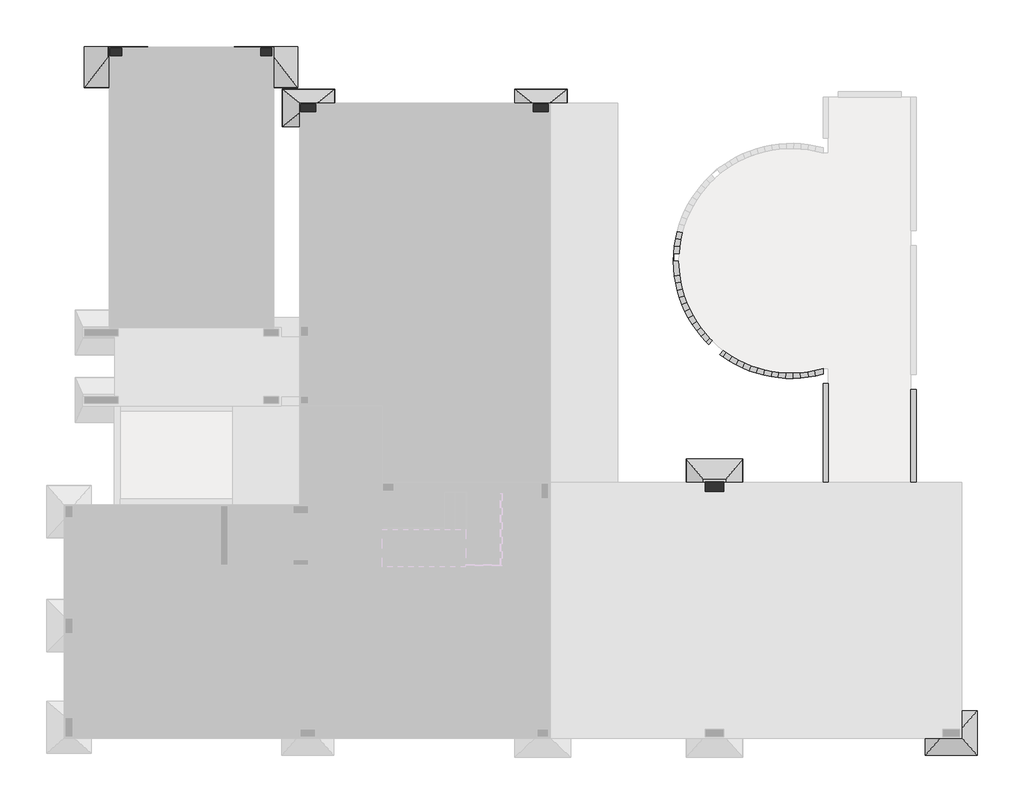
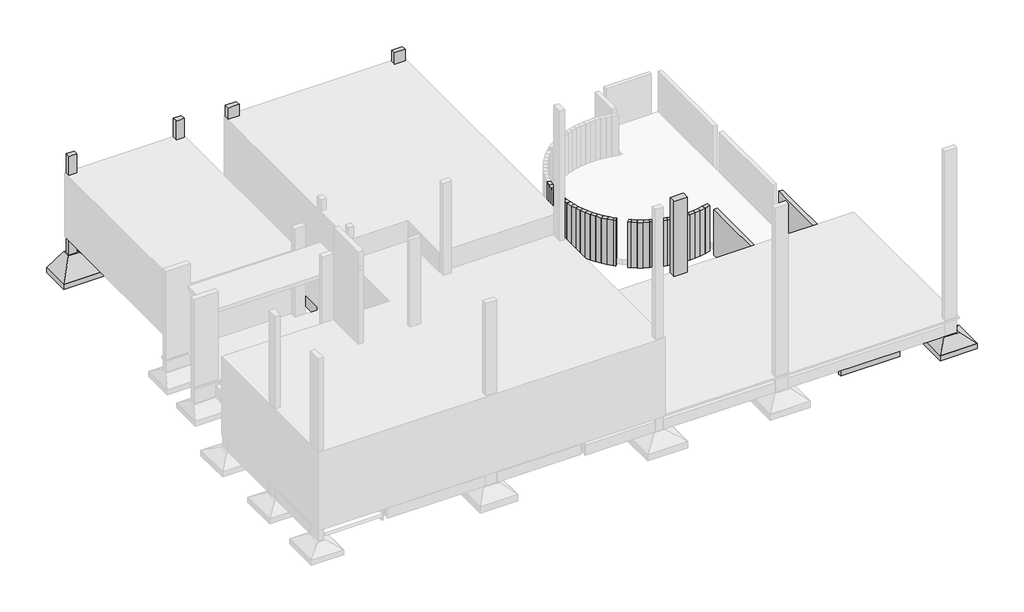
# One storey, part 3 of 4: 37 beams, 7 fasteners, 5 columns.
"""IFC4 building model written with IfcOpenShell, lengths in millimetres."""

import ifcopenshell
import ifcopenshell.guid

model = None  # the IFC model being written
_history = None  # IfcOwnerHistory: only IFC2X3 demands one
_inside = {}  # id of a spatial element -> (the spatial element, [elements in it])
_under = {}  # id of a project, library or spatial element -> (it, [spatial elements below it])
_declared = {}  # id of a project -> (the project, [libraries it declares])
_typed = {}  # id of a type object -> (the type object, [elements of that type])
_made_of = {}  # id of a material, layer set ... -> (it, [elements and type objects made of it])


def new_model(schema):
    """Start an empty IFC model of exactly this schema.

    Asked for "IFC4X3", IfcOpenShell would pick the latest addendum, in which some entities
    have other attributes; the version numbers below select the first issue.
    IFC2X3 requires an IfcOwnerHistory on every rooted entity: one is made here for all.
    """
    global model, _history
    if schema == "IFC4X3":
        model = ifcopenshell.file(schema_version=(4, 3, 0, 0))
    else:
        model = ifcopenshell.file(schema=schema)
    _inside.clear()
    _under.clear()
    _declared.clear()
    _typed.clear()
    _made_of.clear()
    _history = None
    if model.schema == "IFC2X3":
        org = make("IfcOrganization", Name="unknown")
        user = make(
            "IfcPersonAndOrganization",
            ThePerson=make("IfcPerson", FamilyName="unknown"),
            TheOrganization=org,
        )
        app = make(
            "IfcApplication",
            ApplicationDeveloper=org,
            Version="unknown",
            ApplicationFullName="unknown",
            ApplicationIdentifier="unknown",
        )
        _history = make(
            "IfcOwnerHistory",
            OwningUser=user,
            OwningApplication=app,
            ChangeAction="ADDED",
            CreationDate=0,
        )
    return model


def make(cls, **values):
    """One entity of the class cls with the attributes given. An attribute that is None is left unset."""
    return model.create_entity(
        cls, **{name: value for name, value in values.items() if value is not None}
    )


def rooted(cls, **values):
    """An entity with a GlobalId (a new one), such as an element, a storey or a relation."""
    return make(cls, GlobalId=ifcopenshell.guid.new(), OwnerHistory=_history, **values)


def si_unit(unit_type, name, prefix=None):
    """IfcSIUnit, for example si_unit("LENGTHUNIT", "METRE", prefix="MILLI")."""
    return make("IfcSIUnit", UnitType=unit_type, Prefix=prefix, Name=name)


def assignment(units):
    """IfcUnitAssignment: the units of a project."""
    return None if units is None else make("IfcUnitAssignment", Units=units)


def point(xyz):
    """IfcCartesianPoint."""
    return None if xyz is None else make("IfcCartesianPoint", Coordinates=xyz)


def direction(xyz):
    """IfcDirection."""
    return None if xyz is None else make("IfcDirection", DirectionRatios=xyz)


def frame(location, z_axis=None, x_axis=None):
    """IfcAxis2Placement3D, a coordinate frame: its origin and axes. An axis left out is left unset."""
    return make(
        "IfcAxis2Placement3D",
        Location=point(location),
        Axis=direction(z_axis),
        RefDirection=direction(x_axis),
    )


def frame_2d(location, x_axis=None):
    """IfcAxis2Placement2D, a coordinate frame in the plane: its origin and x axis."""
    return make(
        "IfcAxis2Placement2D", Location=point(location), RefDirection=direction(x_axis)
    )


def origin():
    """The frame at (0, 0, 0) with its axes left unset."""
    return frame((0.0, 0.0, 0.0))


def place(relative_to, where):
    """IfcLocalPlacement: puts the frame where relative to a parent placement (None: the world)."""
    return make(
        "IfcLocalPlacement", PlacementRelTo=relative_to, RelativePlacement=where
    )


def context(
    kind, dimensions, precision=None, world=None, true_north=None, identifier=None
):
    """IfcGeometricRepresentationContext, for example the 3D "Model" context."""
    return make(
        "IfcGeometricRepresentationContext",
        ContextIdentifier=identifier,
        ContextType=kind,
        CoordinateSpaceDimension=dimensions,
        Precision=precision,
        WorldCoordinateSystem=world,
        TrueNorth=true_north,
    )


def project(units=None, contexts=None):
    """IfcProject with its units and contexts."""
    return rooted(
        "IfcProject",
        Name="project",
        RepresentationContexts=contexts,
        UnitsInContext=assignment(units),
    )


def spatial(cls, under=None, at=None, **own):
    """A site, building, storey or space (cls), placed at a placement, below another one or the project."""
    s = rooted(cls, ObjectPlacement=at, **own)
    if under is not None:
        _under.setdefault(under.id(), (under, []))[1].append(s)
    return s


def polyline(points):
    """IfcPolyline through the points."""
    return make("IfcPolyline", Points=[point(p) for p in points])


def circle_curve(where, radius):
    """IfcCircle in the frame where."""
    return make("IfcCircle", Position=where, Radius=radius)


def trimmed(basis, trim1, trim2, sense, master):
    """IfcTrimmedCurve: the piece of a basis curve between two trims."""
    return make(
        "IfcTrimmedCurve",
        BasisCurve=basis,
        Trim1=trim1,
        Trim2=trim2,
        SenseAgreement=sense,
        MasterRepresentation=master,
    )


def segment(curve, same_sense, transition):
    """IfcCompositeCurveSegment."""
    return make(
        "IfcCompositeCurveSegment",
        Transition=transition,
        SameSense=same_sense,
        ParentCurve=curve,
    )


def composite_curve(segments, self_intersect=None):
    """IfcCompositeCurve: segments joined end to end."""
    return make("IfcCompositeCurve", Segments=segments, SelfIntersect=self_intersect)


def outline(outer, holes=None, kind="AREA"):
    """IfcArbitraryClosedProfileDef: a profile drawn as a closed curve; with holes, ...WithVoids."""
    if holes is None:
        return make("IfcArbitraryClosedProfileDef", ProfileType=kind, OuterCurve=outer)
    return make(
        "IfcArbitraryProfileDefWithVoids",
        ProfileType=kind,
        OuterCurve=outer,
        InnerCurves=holes,
    )


def extrude(swept, where, along, depth):
    """IfcExtrudedAreaSolid: the profile swept, set in the frame where, extruded along a direction by depth."""
    return make(
        "IfcExtrudedAreaSolid",
        SweptArea=swept,
        Position=where,
        ExtrudedDirection=direction(along),
        Depth=depth,
    )


def faces_of(points, faces, orient=None, outer=None):
    """IfcFace entities. A face is a list of loops; a loop is a list of indices into points, from 0.

    orient and outer hold one flag for each loop. By default every Orientation is true, the
    first loop of a face is its IfcFaceOuterBound and the others are IfcFaceBound.
    """
    made = []
    for i, loops in enumerate(faces):
        bounds = []
        for j, loop in enumerate(loops):
            is_outer = j == 0 if outer is None else outer[i][j]
            bounds.append(
                make(
                    "IfcFaceOuterBound" if is_outer else "IfcFaceBound",
                    Bound=make("IfcPolyLoop", Polygon=[points[k] for k in loop]),
                    Orientation=True if orient is None else orient[i][j],
                )
            )
        made.append(make("IfcFace", Bounds=bounds))
    return made


def faceted_brep(points, faces, orient=None, outer=None, voids=None):
    """IfcFacetedBrep: a solid bounded by flat faces; with voids (closed shells), ...WithVoids."""
    shared = [point(p) for p in points]
    hull = make("IfcClosedShell", CfsFaces=faces_of(shared, faces, orient, outer))
    if voids is None:
        return make("IfcFacetedBrep", Outer=hull)
    return make(
        "IfcFacetedBrepWithVoids",
        Outer=hull,
        Voids=[
            make(cls, CfsFaces=faces_of(shared, fs, o, b)) for cls, fs, o, b in voids
        ],
    )


def shape(context_of_items, identifier, shape_type, items):
    """IfcShapeRepresentation: the items that make up one representation, for example the "Body"."""
    return make(
        "IfcShapeRepresentation",
        ContextOfItems=context_of_items,
        RepresentationIdentifier=identifier,
        RepresentationType=shape_type,
        Items=items,
    )


def source(mapping_origin, context_of_items, identifier, shape_type, items):
    """IfcRepresentationMap: a shape defined once, which mapped items show again and again."""
    return make(
        "IfcRepresentationMap",
        MappingOrigin=mapping_origin,
        MappedRepresentation=shape(context_of_items, identifier, shape_type, items),
    )


def transform(
    local_origin,
    x_axis=None,
    y_axis=None,
    z_axis=None,
    scale=None,
    scale2=None,
    scale3=None,
    uniform=True,
):
    """IfcCartesianTransformationOperator3D, or its non-uniform kind. x_axis, y_axis, z_axis: its Axis1, 2, 3."""
    if uniform:
        return make(
            "IfcCartesianTransformationOperator3D",
            Axis1=direction(x_axis),
            Axis2=direction(y_axis),
            LocalOrigin=point(local_origin),
            Scale=scale,
            Axis3=direction(z_axis),
        )
    return make(
        "IfcCartesianTransformationOperator3DnonUniform",
        Axis1=direction(x_axis),
        Axis2=direction(y_axis),
        LocalOrigin=point(local_origin),
        Scale=scale,
        Axis3=direction(z_axis),
        Scale2=scale2,
        Scale3=scale3,
    )


def mapped(mapping_source, mapping_target):
    """IfcMappedItem: shows the shape of a source again, moved by a transform."""
    return make(
        "IfcMappedItem", MappingSource=mapping_source, MappingTarget=mapping_target
    )


def made_of(thing, what):
    """Note that an element or type object is made of a material, layer set ...; save() writes the relation."""
    if what is not None:
        _made_of.setdefault(what.id(), (what, []))[1].append(thing)
    return thing


def element(
    cls,
    number,
    at=None,
    inside=None,
    cuts=None,
    type_object=None,
    material=None,
    context=None,
    identifier="Body",
    shape_type=None,
    held_by="IfcProductDefinitionShape",
    body=None,
    shapes=None,
    **own,
):
    """One element of the class cls, such as IfcWall. Its Tag is "e" and its number.

    at: its placement. inside: the storey or other place that contains it. cuts: it is an
    opening in that element (IfcRelVoidsElement). A single representation is given by context,
    identifier, shape_type and body (its items); several are given by shapes. held_by: the class
    of the entity that holds the representations. save() writes the other relations.
    """
    e = rooted(cls, Tag="e%d" % number, ObjectPlacement=at, **own)
    if body is not None:
        shapes = [shape(context, identifier, shape_type, body)]
    if shapes is not None:
        e.Representation = make(held_by, Representations=shapes)
    if inside is not None:
        _inside.setdefault(inside.id(), (inside, []))[1].append(e)
    if cuts is not None:
        rooted(
            "IfcRelVoidsElement", RelatingBuildingElement=cuts, RelatedOpeningElement=e
        )
    if type_object is not None:
        _typed.setdefault(type_object.id(), (type_object, []))[1].append(e)
    return made_of(e, material)


def aggregate(whole, parts):
    """IfcRelAggregates: a whole, such as a stair, and the parts it consists of."""
    return rooted("IfcRelAggregates", RelatingObject=whole, RelatedObjects=parts)


def save(model, path):
    """Write the relations noted so far, then the file.

    IfcRelAggregates (storeys below a building ...), IfcRelContainedInSpatialStructure (elements
    in a storey), IfcRelDefinesByType, IfcRelAssociatesMaterial and IfcRelDeclares: one each for
    every whole, place, type object, material and project.
    """
    for whole, parts in _under.values():
        aggregate(whole, parts)
    for where, things in _inside.values():
        rooted(
            "IfcRelContainedInSpatialStructure",
            RelatedElements=things,
            RelatingStructure=where,
        )
    for kind, things in _typed.values():
        rooted("IfcRelDefinesByType", RelatedObjects=things, RelatingType=kind)
    for what, things in _made_of.values():
        rooted("IfcRelAssociatesMaterial", RelatedObjects=things, RelatingMaterial=what)
    for by, libraries in _declared.values():
        rooted("IfcRelDeclares", RelatingContext=by, RelatedDefinitions=libraries)
    model.write(path)


def tqs_viga_retangular_19_0_x_30_0_29604a85(model_context):
    return source(origin(), model_context, "Body", "SweptSolid", [
        extrude(outline(polyline([(1809.0, 95.0), (1809.0, -95.0), (-1809.0, -95.0), (-1809.0, 95.0), (1809.0, 95.0)])), frame((0.0, 0.0, -150.0), z_axis=(0.0, 0.0, 1.0), x_axis=(1.0, 0.0, 0.0)), (0.0, 0.0, 1.0), 300.0),
    ])


def s1_ccae0304(model_context):
    return source(origin(), model_context, "Body", "SolidModel", [
        faceted_brep([(-460.0, 0.0, 0.0), (-750.0, 0.0, 0.0), (-750.0, -400.0, 0.0), (-460.0, -400.0, 0.0), (350.0, 650.0, -400.0), (350.0, -1050.0, -400.0), (-750.0, -1050.0, -400.0), (-750.0, 650.0, -400.0)], [[[0, 1, 2, 3]], [[4, 5, 6, 7]], [[4, 7, 1, 0]], [[7, 6, 2, 1]], [[6, 5, 3, 2]], [[5, 4, 0, 3]]]),
        extrude(outline(polyline([(350.0, 650.0), (350.0, -1050.0), (-750.0, -1050.0), (-750.0, 650.0), (350.0, 650.0)])), frame((0.0, 0.0, -600.0), z_axis=(0.0, 0.0, 1.0), x_axis=(1.0, 0.0, 0.0)), (0.0, 0.0, 1.0), 200.0),
    ])


def s12_1e6d1b45(model_context):
    return source(origin(), model_context, "Body", "SolidModel", [
        faceted_brep([(-55.0, 50.0, 0.0), (-345.0, 50.0, 0.0), (-345.0, -450.0, 0.0), (-55.0, -450.0, 0.0), (550.0, 550.0, -350.0), (550.0, -950.0, -350.0), (-950.0, -950.0, -350.0), (-950.0, 550.0, -350.0)], [[[0, 1, 2, 3]], [[4, 5, 6, 7]], [[4, 7, 1, 0]], [[7, 6, 2, 1]], [[6, 5, 3, 2]], [[5, 4, 0, 3]]]),
        extrude(outline(polyline([(550.0, 550.0), (550.0, -950.0), (-950.0, -950.0), (-950.0, 550.0), (550.0, 550.0)])), frame((0.0, 0.0, -600.0), z_axis=(0.0, 0.0, 1.0), x_axis=(1.0, 0.0, 0.0)), (0.0, 0.0, 1.0), 250.0),
    ])


def s13_7eae1afe(model_context):
    return source(origin(), model_context, "Body", "SolidModel", [
        faceted_brep([(-5.0, 100.0, 0.0), (-395.0, 100.0, 0.0), (-395.0, -500.0, 0.0), (-5.0, -500.0, 0.0), (550.0, 550.0, -300.0), (550.0, -950.0, -300.0), (-950.0, -950.0, -300.0), (-950.0, 550.0, -300.0)], [[[0, 1, 2, 3]], [[4, 5, 6, 7]], [[4, 7, 1, 0]], [[7, 6, 2, 1]], [[6, 5, 3, 2]], [[5, 4, 0, 3]]]),
        extrude(outline(polyline([(550.0, 550.0), (550.0, -950.0), (-950.0, -950.0), (-950.0, 550.0), (550.0, 550.0)])), frame((0.0, 0.0, -500.0), z_axis=(0.0, 0.0, 1.0), x_axis=(1.0, 0.0, 0.0)), (0.0, 0.0, 1.0), 200.0),
    ])


def s20_c409a0c5(model_context):
    return source(origin(), model_context, "Body", "SolidModel", [
        faceted_brep([(-55.0, 100.0, 0.0), (-345.0, 100.0, 0.0), (-345.0, -500.0, 0.0), (-55.0, -500.0, 0.0), (400.0, 500.0, -300.0), (400.0, -900.0, -300.0), (-800.0, -900.0, -300.0), (-800.0, 500.0, -300.0)], [[[0, 1, 2, 3]], [[4, 5, 6, 7]], [[4, 7, 1, 0]], [[7, 6, 2, 1]], [[6, 5, 3, 2]], [[5, 4, 0, 3]]]),
        extrude(outline(polyline([(400.0, 500.0), (400.0, -900.0), (-800.0, -900.0), (-800.0, 500.0), (400.0, 500.0)])), frame((0.0, 0.0, -500.0), z_axis=(0.0, 0.0, 1.0), x_axis=(1.0, 0.0, 0.0)), (0.0, 0.0, 1.0), 200.0),
    ])


def s3_fc183e28(model_context):
    return source(origin(), model_context, "Body", "SolidModel", [
        faceted_brep([(-55.0, 50.0, 0.0), (-345.0, 50.0, 0.0), (-345.0, -450.0, 0.0), (-55.0, -450.0, 0.0), (300.0, 500.0, -300.0), (300.0, -900.0, -300.0), (-700.0, -900.0, -300.0), (-700.0, 500.0, -300.0)], [[[0, 1, 2, 3]], [[4, 5, 6, 7]], [[4, 7, 1, 0]], [[7, 6, 2, 1]], [[6, 5, 3, 2]], [[5, 4, 0, 3]]]),
        extrude(outline(polyline([(300.0, 500.0), (300.0, -900.0), (-700.0, -900.0), (-700.0, 500.0), (300.0, 500.0)])), frame((0.0, 0.0, -500.0), z_axis=(0.0, 0.0, 1.0), x_axis=(1.0, 0.0, 0.0)), (0.0, 0.0, 1.0), 200.0),
    ])


model = new_model("IFC4")

# Units and contexts
model_context = context("Model", 3, world=origin())
ifc_project = project(units=[si_unit("LENGTHUNIT", "METRE", prefix="MILLI")], contexts=[model_context])

# Site, building, storey
site = spatial("IfcSite", under=ifc_project)
building = spatial("IfcBuilding", under=site)
storey = spatial("IfcBuildingStorey", under=building, Name="PAVIMENTO TÉRREO", Elevation=500.0)

# Beams
placement = place(None, origin())
element("IfcBeam", 1, ObjectType="TQS - Viga retangular : 14.0 x 180.0", at=placement, inside=storey, context=model_context, shape_type="Brep", body=[
    faceted_brep([(9682.718693, -9679.5699847, 350.0), (9682.718693, -9539.5699847, 350.0), (7474.718693, -9539.5699847, 350.0), (7474.718693, -9679.5699847, 350.0), (9682.718693, -9679.5699847, -1450.0), (7474.718693, -9679.5699847, -1450.0), (9682.718693, -9539.5699847, -1450.0), (7474.718693, -9539.5699847, -1450.0), (9682.718693, -9539.5699847, -1250.0), (7474.718693, -9539.5699847, -1250.0)], [[[0, 1, 2, 3]], [[4, 0, 3, 5]], [[6, 4, 5, 7]], [[1, 8, 6, 7, 9, 2]], [[2, 9, 7, 5, 3]], [[1, 0, 4, 6, 8]]]),
])
element("IfcBeam", 2, ObjectType="TQS - Viga retangular : 14.0 x 180.0", at=placement, inside=storey, context=model_context, shape_type="Brep", body=[
    faceted_brep([(7474.718693, -1696.0936198, 350.0), (7334.718693, -1696.0936198, 350.0), (7334.718693, -5230.1494451, 350.0), (7474.718693, -5230.1494451, 350.0), (7474.718693, -5230.1494451, -1250.0), (7474.718693, -5230.1494451, -1450.0), (7474.718693, -1696.0936198, -1450.0), (7474.718693, -1696.0936198, -1250.0), (7334.718693, -1696.0936198, -1450.0), (7334.718693, -5230.1494451, -1450.0)], [[[0, 1, 2, 3]], [[0, 3, 4, 5, 6, 7]], [[8, 6, 5, 9]], [[1, 8, 9, 2]], [[1, 0, 7, 6, 8]], [[3, 2, 9, 5, 4]]]),
    faceted_brep([(7334.718693, -5630.1494451, 350.0), (7474.718693, -5630.1494451, 350.0), (7474.718693, -5630.1494451, -1250.0), (7474.718693, -5630.1494451, -1450.0), (7334.718693, -5630.1494451, -1450.0), (7334.718693, -9279.5699847, 350.0), (7474.718693, -9279.5699847, 350.0), (7474.718693, -9279.5699847, -1250.0), (7474.718693, -9279.5699847, -1450.0), (7334.718693, -9279.5699847, -1450.0)], [[[0, 1, 2, 3, 4]], [[1, 0, 5, 6]], [[1, 6, 7, 8, 3, 2]], [[4, 3, 8, 9]], [[0, 4, 9, 5]], [[6, 5, 9, 8, 7]]]),
])
element("IfcBeam", 3, ObjectType="TQS - Viga retangular : 14.0 x 180.0", at=placement, inside=storey, context=model_context, shape_type="Brep", body=[
    faceted_brep([(7334.718693, -1296.0936198, 350.0), (7106.1277936, -1352.3610531, 350.0), (7135.2990206, -1489.35947, 350.0), (7334.718693, -1440.2725066, 350.0), (7334.718693, -1296.0936198, -1250.0), (7334.718693, -1296.0936198, -1450.0), (7106.1277936, -1352.3610531, -1450.0), (7106.1277936, -1352.3610531, -1250.0), (7334.718693, -1440.2725066, -1450.0), (7135.2990206, -1489.35947, -1450.0)], [[[0, 1, 2, 3]], [[1, 0, 4, 5, 6, 7]], [[6, 5, 8, 9]], [[3, 2, 9, 8]], [[0, 3, 8, 5, 4]], [[2, 1, 7, 6, 9]]]),
])
element("IfcBeam", 4, ObjectType="TQS - Viga retangular : 14.0 x 180.0", at=placement, inside=storey, context=model_context, shape_type="Brep", body=[
    faceted_brep([(6938.2242767, -1524.8638101, 350.0), (7135.2990206, -1489.35947, 350.0), (7106.1277936, -1352.3610531, 350.0), (6917.7849868, -1386.2922761, 350.0), (7106.1277936, -1352.3610531, -1250.0), (7106.1277936, -1352.3610531, -1450.0), (6917.7849868, -1386.2922761, -1450.0), (6917.7849868, -1386.2922761, -1250.0), (7135.2990206, -1489.35947, -1450.0), (6938.2242767, -1524.8638101, -1450.0)], [[[0, 1, 2, 3]], [[3, 2, 4, 5, 6, 7]], [[6, 5, 8, 9]], [[1, 0, 9, 8]], [[1, 8, 5, 4, 2]], [[0, 3, 7, 6, 9]]]),
])
element("IfcBeam", 5, ObjectType="TQS - Viga retangular : 14.0 x 180.0", at=placement, inside=storey, context=model_context, shape_type="Brep", body=[
    faceted_brep([(6739.2913899, -1547.770563, 350.0), (6938.2242767, -1524.8638101, 350.0), (6917.7849868, -1386.2922761, 350.0), (6727.7008432, -1408.1801126, 350.0), (6917.7849868, -1386.2922761, -1250.0), (6917.7849868, -1386.2922761, -1450.0), (6727.7008432, -1408.1801126, -1450.0), (6727.7008432, -1408.1801126, -1250.0), (6938.2242767, -1524.8638101, -1450.0), (6739.2913899, -1547.770563, -1450.0)], [[[0, 1, 2, 3]], [[3, 2, 4, 5, 6, 7]], [[6, 5, 8, 9]], [[1, 0, 9, 8]], [[1, 8, 5, 4, 2]], [[0, 3, 7, 6, 9]]]),
])
element("IfcBeam", 6, ObjectType="TQS - Viga retangular : 14.0 x 180.0", at=placement, inside=storey, context=model_context, shape_type="Brep", body=[
    faceted_brep([(6539.3048029, -1557.9870986, 350.0), (6739.2913899, -1547.770563, 350.0), (6727.7008432, -1408.1801126, 350.0), (6536.6098693, -1417.942206, 350.0), (6727.7008432, -1408.1801126, -1250.0), (6727.7008432, -1408.1801126, -1450.0), (6536.6098693, -1417.942206, -1450.0), (6536.6098693, -1417.942206, -1250.0), (6739.2913899, -1547.770563, -1450.0), (6539.3048029, -1557.9870986, -1450.0)], [[[0, 1, 2, 3]], [[3, 2, 4, 5, 6, 7]], [[6, 5, 8, 9]], [[1, 0, 9, 8]], [[1, 8, 5, 4, 2]], [[0, 3, 7, 6, 9]]]),
])
element("IfcBeam", 7, ObjectType="TQS - Viga retangular : 14.0 x 180.0", at=placement, inside=storey, context=model_context, shape_type="Brep", body=[
    faceted_brep([(6339.0732182, -1555.4721035, 350.0), (6539.3048029, -1557.9870986, 350.0), (6536.6098693, -1417.942206, 350.0), (6345.2847953, -1415.5390805, 350.0), (6536.6098693, -1417.942206, -1250.0), (6536.6098693, -1417.942206, -1450.0), (6345.2847953, -1415.5390805, -1450.0), (6345.2847953, -1415.5390805, -1250.0), (6539.3048029, -1557.9870986, -1450.0), (6339.0732182, -1555.4721035, -1450.0)], [[[0, 1, 2, 3]], [[3, 2, 4, 5, 6, 7]], [[6, 5, 8, 9]], [[1, 0, 9, 8]], [[1, 8, 5, 4, 2]], [[0, 3, 7, 6, 9]]]),
])
element("IfcBeam", 8, ObjectType="TQS - Viga retangular : 14.0 x 180.0", at=placement, inside=storey, context=model_context, shape_type="Brep", body=[
    faceted_brep([(6139.4063301, -1540.2357477, 350.0), (6339.0732182, -1555.4721035, 350.0), (6345.2847953, -1415.5390805, 350.0), (6154.4732894, -1400.978469, 350.0), (6345.2847953, -1415.5390805, -1250.0), (6345.2847953, -1415.5390805, -1450.0), (6154.4732894, -1400.978469, -1450.0), (6154.4732894, -1400.978469, -1250.0), (6339.0732182, -1555.4721035, -1450.0), (6139.4063301, -1540.2357477, -1450.0)], [[[0, 1, 2, 3]], [[3, 2, 4, 5, 6, 7]], [[6, 5, 8, 9]], [[1, 0, 9, 8]], [[1, 8, 5, 4, 2]], [[0, 3, 7, 6, 9]]]),
])
element("IfcBeam", 9, ObjectType="TQS - Viga retangular : 14.0 x 180.0", at=placement, inside=storey, context=model_context, shape_type="Brep", body=[
    faceted_brep([(5942.253541, -1512.5751442, 350.0), (6139.4063301, -1540.2357477, 350.0), (6154.4732894, -1400.978469, 350.0), (5966.1413215, -1374.5554297, 350.0), (6154.4732894, -1400.978469, -1250.0), (6154.4732894, -1400.978469, -1450.0), (5966.1413215, -1374.5554297, -1450.0), (5966.1413215, -1374.5554297, -1250.0), (6139.4063301, -1540.2357477, -1450.0), (5942.253541, -1512.5751442, -1450.0)], [[[0, 1, 2, 3]], [[3, 2, 4, 5, 6, 7]], [[6, 5, 8, 9]], [[1, 0, 9, 8]], [[1, 8, 5, 4, 2]], [[0, 3, 7, 6, 9]]]),
])
element("IfcBeam", 10, ObjectType="TQS - Viga retangular : 14.0 x 180.0", at=placement, inside=storey, context=model_context, shape_type="Brep", body=[
    faceted_brep([(5746.1327296, -1472.1320983, 350.0), (5942.253541, -1512.5751442, 350.0), (5966.1413215, -1374.5554297, 350.0), (5778.7697179, -1335.9166013, 350.0), (5966.1413215, -1374.5554297, -1250.0), (5966.1413215, -1374.5554297, -1450.0), (5778.7697179, -1335.9166013, -1450.0), (5778.7697179, -1335.9166013, -1250.0), (5942.253541, -1512.5751442, -1450.0), (5746.1327296, -1472.1320983, -1450.0)], [[[0, 1, 2, 3]], [[3, 2, 4, 5, 6, 7]], [[6, 5, 8, 9]], [[1, 0, 9, 8]], [[1, 8, 5, 4, 2]], [[0, 3, 7, 6, 9]]]),
])
element("IfcBeam", 11, ObjectType="TQS - Viga retangular : 14.0 x 180.0", at=placement, inside=storey, context=model_context, shape_type="Brep", body=[
    faceted_brep([(5552.9789583, -1419.3056534, 350.0), (5746.1327296, -1472.1320983, 350.0), (5778.7697179, -1335.9166013, 350.0), (5594.2076289, -1285.4399321, 350.0), (5778.7697179, -1335.9166013, -1250.0), (5778.7697179, -1335.9166013, -1450.0), (5594.2076289, -1285.4399321, -1450.0), (5594.2076289, -1285.4399321, -1250.0), (5746.1327296, -1472.1320983, -1450.0), (5552.9789583, -1419.3056534, -1450.0)], [[[0, 1, 2, 3]], [[3, 2, 4, 5, 6, 7]], [[6, 5, 8, 9]], [[1, 0, 9, 8]], [[1, 8, 5, 4, 2]], [[0, 3, 7, 6, 9]]]),
])
element("IfcBeam", 12, ObjectType="TQS - Viga retangular : 14.0 x 180.0", at=placement, inside=storey, context=model_context, shape_type="Brep", body=[
    faceted_brep([(5363.9986658, -1354.4553965, 350.0), (5552.9789583, -1419.3056534, 350.0), (5594.2076289, -1285.4399321, 350.0), (5413.6522985, -1223.4807754, 350.0), (5594.2076289, -1285.4399321, -1250.0), (5594.2076289, -1285.4399321, -1450.0), (5413.6522985, -1223.4807754, -1450.0), (5413.6522985, -1223.4807754, -1250.0), (5552.9789583, -1419.3056534, -1450.0), (5363.9986658, -1354.4553965, -1450.0)], [[[0, 1, 2, 3]], [[3, 2, 4, 5, 6, 7]], [[6, 5, 8, 9]], [[1, 0, 9, 8]], [[1, 8, 5, 4, 2]], [[0, 3, 7, 6, 9]]]),
])
element("IfcBeam", 13, ObjectType="TQS - Viga retangular : 14.0 x 180.0", at=placement, inside=storey, context=model_context, shape_type="Brep", body=[
    faceted_brep([(5179.1069104, -1277.5521698, 350.0), (5363.9986658, -1354.4553965, 350.0), (5413.6522985, -1223.4807754, 350.0), (5236.9847165, -1149.9982825, 350.0), (5413.6522985, -1223.4807754, -1250.0), (5413.6522985, -1223.4807754, -1450.0), (5236.9847165, -1149.9982825, -1450.0), (5236.9847165, -1149.9982825, -1250.0), (5363.9986658, -1354.4553965, -1450.0), (5179.1069104, -1277.5521698, -1450.0)], [[[0, 1, 2, 3]], [[3, 2, 4, 5, 6, 7]], [[6, 5, 8, 9]], [[1, 0, 9, 8]], [[1, 8, 5, 4, 2]], [[0, 3, 7, 6, 9]]]),
])
element("IfcBeam", 14, ObjectType="TQS - Viga retangular : 14.0 x 180.0", at=placement, inside=storey, context=model_context, shape_type="Brep", body=[
    faceted_brep([(4999.4769736, -1189.0530269, 350.0), (5179.1069104, -1277.5521698, 350.0), (5236.9847165, -1149.9982825, 350.0), (5065.344906, -1065.4356735, 350.0), (5236.9847165, -1149.9982825, -1250.0), (5236.9847165, -1149.9982825, -1450.0), (5065.344906, -1065.4356735, -1450.0), (5065.344906, -1065.4356735, -1250.0), (5179.1069104, -1277.5521698, -1450.0), (4999.4769736, -1189.0530269, -1450.0)], [[[0, 1, 2, 3]], [[3, 2, 4, 5, 6, 7]], [[6, 5, 8, 9]], [[1, 0, 9, 8]], [[1, 8, 5, 4, 2]], [[0, 3, 7, 6, 9]]]),
])
element("IfcBeam", 15, ObjectType="TQS - Viga retangular : 14.0 x 180.0", at=placement, inside=storey, context=model_context, shape_type="Brep", body=[
    faceted_brep([(4825.8347061, -1089.3155581, 350.0), (4999.4769736, -1189.0530269, 350.0), (5065.344906, -1065.4356735, 350.0), (4899.4264221, -970.1346281, 350.0), (5065.344906, -1065.4356735, -1250.0), (5065.344906, -1065.4356735, -1450.0), (4899.4264221, -970.1346281, -1450.0), (4899.4264221, -970.1346281, -1250.0), (4999.4769736, -1189.0530269, -1450.0), (4825.8347061, -1089.3155581, -1450.0)], [[[0, 1, 2, 3]], [[3, 2, 4, 5, 6, 7]], [[6, 5, 8, 9]], [[1, 0, 9, 8]], [[1, 8, 5, 4, 2]], [[0, 3, 7, 6, 9]]]),
])
element("IfcBeam", 16, ObjectType="TQS - Viga retangular : 14.0 x 180.0", at=placement, inside=storey, context=model_context, shape_type="Brep", body=[
    faceted_brep([(4659.7082838, -979.2900143, 350.0), (4825.8347061, -1089.3155581, 350.0), (4899.4264221, -970.1346281, 350.0), (4740.8701617, -865.1228032, 350.0), (4899.4264221, -970.1346281, -1250.0), (4899.4264221, -970.1346281, -1450.0), (4740.8701617, -865.1228032, -1450.0), (4740.8701617, -865.1228032, -1250.0), (4825.8347061, -1089.3155581, -1450.0), (4659.7082838, -979.2900143, -1450.0)], [[[0, 1, 2, 3]], [[3, 2, 4, 5, 6, 7]], [[6, 5, 8, 9]], [[1, 0, 9, 8]], [[1, 8, 5, 4, 2]], [[0, 3, 7, 6, 9]]]),
])
element("IfcBeam", 17, ObjectType="TQS - Viga retangular : 14.0 x 180.0", at=placement, inside=storey, context=model_context, shape_type="Brep", body=[
    faceted_brep([(4571.9800682, -912.4546637, 350.0), (4659.7082838, -979.2900143, 350.0), (4740.8701617, -865.1228032, 350.0), (4665.976342, -808.0652799, 350.0), (4740.8701617, -865.1228032, -1250.0), (4740.8701617, -865.1228032, -1450.0), (4665.976342, -808.0652799, -1450.0), (4665.976342, -808.0652799, -1250.0), (4659.7082838, -979.2900143, -1450.0), (4571.9800682, -912.4546637, -1450.0)], [[[0, 1, 2, 3]], [[3, 2, 4, 5, 6, 7]], [[8, 9, 6, 5]], [[1, 0, 9, 8]], [[0, 3, 7, 6, 9]], [[1, 8, 5, 4, 2]]]),
])
element("IfcBeam", 18, ObjectType="TQS - Viga retangular : 14.0 x 180.0", at=placement, inside=storey, context=model_context, shape_type="Brep", body=[
    faceted_brep([(4206.3905749, -587.9275531, 350.0), (4270.2869357, -650.1191423, 350.0), (4367.9344995, -549.7949015, 350.0), (4307.4254093, -490.9002096, 350.0), (4367.9344995, -549.7949015, -1450.0), (4362.9503182, -544.9436994, -1450.0), (4307.4254093, -490.9002096, -1450.0), (4307.4254093, -490.9002096, -1250.0), (4270.2869357, -650.1191423, -1450.0), (4206.3905749, -587.9275531, -1450.0)], [[[0, 1, 2, 3]], [[3, 2, 4, 5, 6, 7]], [[8, 9, 6, 5, 4]], [[1, 0, 9, 8]], [[1, 8, 4, 2]], [[0, 3, 7, 6, 9]]]),
])
element("IfcBeam", 19, ObjectType="TQS - Viga retangular : 14.0 x 180.0", at=placement, inside=storey, context=model_context, shape_type="Brep", body=[
    faceted_brep([(4072.6403676, -438.8977092, 350.0), (4206.3905749, -587.9275531, 350.0), (4307.4254093, -490.9002096, 350.0), (4179.8070625, -348.7027306, 350.0), (4307.4254093, -490.9002096, -1250.0), (4307.4254093, -490.9002096, -1450.0), (4179.8070625, -348.7027306, -1450.0), (4179.8070625, -348.7027306, -1250.0), (4206.3905749, -587.9275531, -1450.0), (4072.6403676, -438.8977092, -1450.0)], [[[0, 1, 2, 3]], [[3, 2, 4, 5, 6, 7]], [[6, 5, 8, 9]], [[1, 0, 9, 8]], [[1, 8, 5, 4, 2]], [[0, 3, 7, 6, 9]]]),
])
element("IfcBeam", 20, ObjectType="TQS - Viga retangular : 14.0 x 180.0", at=placement, inside=storey, context=model_context, shape_type="Brep", body=[
    faceted_brep([(3949.2502321, -282.451126, 350.0), (4072.6403676, -438.8977092, 350.0), (4179.8070625, -348.7027306, 350.0), (4061.9329165, -199.2498808, 350.0), (4179.8070625, -348.7027306, -1250.0), (4179.8070625, -348.7027306, -1450.0), (4061.9329165, -199.2498808, -1450.0), (4061.9329165, -199.2498808, -1250.0), (4072.6403676, -438.8977092, -1450.0), (3949.2502321, -282.451126, -1450.0)], [[[0, 1, 2, 3]], [[3, 2, 4, 5, 6, 7]], [[6, 5, 8, 9]], [[1, 0, 9, 8]], [[1, 8, 5, 4, 2]], [[0, 3, 7, 6, 9]]]),
])
element("IfcBeam", 21, ObjectType="TQS - Viga retangular : 14.0 x 180.0", at=placement, inside=storey, context=model_context, shape_type="Brep", body=[
    faceted_brep([(3835.4866089, -117.6577696, 350.0), (3949.2502321, -282.451126, 350.0), (4061.9329165, -199.2498808, 350.0), (3953.2296156, -41.7867013, 350.0), (4061.9329165, -199.2498808, -1250.0), (4061.9329165, -199.2498808, -1450.0), (3953.2296156, -41.7867013, -1450.0), (3953.2296156, -41.7867013, -1250.0), (3949.2502321, -282.451126, -1450.0), (3835.4866089, -117.6577696, -1450.0)], [[[0, 1, 2, 3]], [[3, 2, 4, 5, 6, 7]], [[6, 5, 8, 9]], [[1, 0, 9, 8]], [[1, 8, 5, 4, 2]], [[0, 3, 7, 6, 9]]]),
])
element("IfcBeam", 22, ObjectType="TQS - Viga retangular : 14.0 x 180.0", at=placement, inside=storey, context=model_context, shape_type="Brep", body=[
    faceted_brep([(3732.4270441, 54.0330523, 350.0), (3835.4866089, -117.6577696, 350.0), (3953.2296156, -41.7867013, 350.0), (3854.7542482, 122.2671329, 350.0), (3953.2296156, -41.7867013, -1250.0), (3953.2296156, -41.7867013, -1450.0), (3854.7542482, 122.2671329, -1450.0), (3854.7542482, 122.2671329, -1250.0), (3835.4866089, -117.6577696, -1450.0), (3732.4270441, 54.0330523, -1450.0)], [[[0, 1, 2, 3]], [[3, 2, 4, 5, 6, 7]], [[6, 5, 8, 9]], [[1, 0, 9, 8]], [[1, 8, 5, 4, 2]], [[0, 3, 7, 6, 9]]]),
])
element("IfcBeam", 23, ObjectType="TQS - Viga retangular : 14.0 x 180.0", at=placement, inside=storey, context=model_context, shape_type="Brep", body=[
    faceted_brep([(3640.48809, 231.9274426, 350.0), (3732.4270441, 54.0330523, 350.0), (3854.7542482, 122.2671329, 350.0), (3766.9048318, 292.2486007, 350.0), (3854.7542482, 122.2671329, -1250.0), (3854.7542482, 122.2671329, -1450.0), (3766.9048318, 292.2486007, -1450.0), (3766.9048318, 292.2486007, -1250.0), (3732.4270441, 54.0330523, -1450.0), (3640.48809, 231.9274426, -1450.0)], [[[0, 1, 2, 3]], [[3, 2, 4, 5, 6, 7]], [[6, 5, 8, 9]], [[1, 0, 9, 8]], [[1, 8, 5, 4, 2]], [[0, 3, 7, 6, 9]]]),
])
element("IfcBeam", 24, ObjectType="TQS - Viga retangular : 14.0 x 180.0", at=placement, inside=storey, context=model_context, shape_type="Brep", body=[
    faceted_brep([(3560.3661231, 414.5663391, 350.0), (3640.48809, 231.9274426, 350.0), (3766.9048318, 292.2486007, 350.0), (3690.3611932, 466.7306588, 350.0), (3766.9048318, 292.2486007, -1250.0), (3766.9048318, 292.2486007, -1450.0), (3690.3611932, 466.7306588, -1450.0), (3690.3611932, 466.7306588, -1250.0), (3640.48809, 231.9274426, -1450.0), (3560.3661231, 414.5663391, -1450.0)], [[[0, 1, 2, 3]], [[3, 2, 4, 5, 6, 7]], [[6, 5, 8, 9]], [[1, 0, 9, 8]], [[1, 8, 5, 4, 2]], [[0, 3, 7, 6, 9]]]),
])
element("IfcBeam", 25, ObjectType="TQS - Viga retangular : 14.0 x 180.0", at=placement, inside=storey, context=model_context, shape_type="Brep", body=[
    faceted_brep([(3491.737855, 602.6864416, 350.0), (3560.3661231, 414.5663391, 350.0), (3690.3611932, 466.7306588, 350.0), (3624.7902852, 646.4700908, 350.0), (3690.3611932, 466.7306588, -1250.0), (3690.3611932, 466.7306588, -1450.0), (3624.7902852, 646.4700908, -1450.0), (3624.7902852, 646.4700908, -1250.0), (3560.3661231, 414.5663391, -1450.0), (3491.737855, 602.6864416, -1450.0)], [[[0, 1, 2, 3]], [[3, 2, 4, 5, 6, 7]], [[6, 5, 8, 9]], [[1, 0, 9, 8]], [[1, 8, 5, 4, 2]], [[0, 3, 7, 6, 9]]]),
])
element("IfcBeam", 26, ObjectType="TQS - Viga retangular : 14.0 x 180.0", at=placement, inside=storey, context=model_context, shape_type="Brep", body=[
    faceted_brep([(3435.4159463, 794.2099051, 350.0), (3491.737855, 602.6864416, 350.0), (3624.7902852, 646.4700908, 350.0), (3570.9813422, 829.4481782, 350.0), (3624.7902852, 646.4700908, -1250.0), (3624.7902852, 646.4700908, -1450.0), (3570.9813422, 829.4481782, -1450.0), (3570.9813422, 829.4481782, -1250.0), (3491.737855, 602.6864416, -1450.0), (3435.4159463, 794.2099051, -1450.0)], [[[0, 1, 2, 3]], [[3, 2, 4, 5, 6, 7]], [[6, 5, 8, 9]], [[1, 0, 9, 8]], [[1, 8, 5, 4, 2]], [[0, 3, 7, 6, 9]]]),
])
element("IfcBeam", 27, ObjectType="TQS - Viga retangular : 14.0 x 180.0", at=placement, inside=storey, context=model_context, shape_type="Brep", body=[
    faceted_brep([(3391.2071159, 989.5163089, 350.0), (3435.4159463, 794.2099051, 350.0), (3570.9813422, 829.4481782, 350.0), (3528.735935, 1016.0805429, 350.0), (3570.9813422, 829.4481782, -1250.0), (3570.9813422, 829.4481782, -1450.0), (3528.735935, 1016.0805429, -1450.0), (3528.735935, 1016.0805429, -1250.0), (3435.4159463, 794.2099051, -1450.0), (3391.2071159, 989.5163089, -1450.0)], [[[0, 1, 2, 3]], [[3, 2, 4, 5, 6, 7]], [[6, 5, 8, 9]], [[1, 0, 9, 8]], [[1, 8, 5, 4, 2]], [[0, 3, 7, 6, 9]]]),
])
element("IfcBeam", 28, ObjectType="TQS - Viga retangular : 14.0 x 180.0", at=placement, inside=storey, context=model_context, shape_type="Brep", body=[
    faceted_brep([(3359.6001228, 1186.6200486, 350.0), (3391.2071159, 989.5163089, 350.0), (3528.735935, 1016.0805429, 350.0), (3498.5672214, 1204.2150568, 350.0), (3528.735935, 1016.0805429, -1250.0), (3528.735935, 1016.0805429, -1450.0), (3498.5672214, 1204.2150568, -1450.0), (3498.5672214, 1204.2150568, -1250.0), (3391.2071159, 989.5163089, -1450.0), (3359.6001228, 1186.6200486, -1450.0)], [[[0, 1, 2, 3]], [[3, 2, 4, 5, 6, 7]], [[6, 5, 8, 9]], [[1, 0, 9, 8]], [[1, 8, 5, 4, 2]], [[0, 3, 7, 6, 9]]]),
])
element("IfcBeam", 29, ObjectType="TQS - Viga retangular : 14.0 x 180.0", at=placement, inside=storey, context=model_context, shape_type="Brep", body=[
    faceted_brep([(3322.4683621, 1585.2441839, 350.0), (3359.6001228, 1186.6200486, 350.0), (3498.5672214, 1204.2150568, 350.0), (3463.0733079, 1585.2562551, 350.0), (3335.9283808, 1585.2453395, 350.0), (3498.5672214, 1204.2150568, -1250.0), (3498.5672214, 1204.2150568, -1450.0), (3481.6870042, 1385.4308636, -1450.0), (3463.0733079, 1585.2562551, -1450.0), (3359.6001228, 1186.6200486, -1450.0), (3322.4683621, 1585.2441839, -1450.0), (3335.9283808, 1585.2453395, -1450.0)], [[[0, 1, 2, 3, 4]], [[3, 2, 5, 6, 7, 8]], [[9, 10, 11, 8, 7, 6]], [[1, 0, 10, 9]], [[0, 4, 3, 8, 11, 10]], [[1, 9, 6, 5, 2]]]),
])
element("IfcBeam", 30, ObjectType="TQS - Viga retangular : 14.0 x 180.0", at=placement, inside=storey, context=model_context, shape_type="SweptSolid", body=[
    extrude(outline(polyline([(3322.4683621, 1585.2441839), (3359.6197005, 1984.821412), (3498.5878389, 1967.228978), (3481.5501681, 1783.9821402), (3342.1096921, 1786.0821852), (3335.8794834, 1590.2360081), (3335.9283808, 1585.2453395), (3322.4683621, 1585.2441839)])), frame((0.0, 0.0, -1450.0), z_axis=(0.0, 0.0, 1.0), x_axis=(1.0, 0.0, 0.0)), (0.0, 0.0, 1.0), 1800.0),
])
element("IfcBeam", 31, ObjectType="TQS - Viga retangular : 14.0 x 180.0", at=placement, inside=storey, context=model_context, shape_type="Brep", body=[
    faceted_brep([(3391.2860591, 2182.1270296, 350.0), (3359.6197005, 1984.821412, 350.0), (3498.5878389, 1967.228978, 350.0), (3528.8128087, 2155.5536418, 350.0), (3498.5878389, 1967.228978, -1250.0), (3498.5878389, 1967.228978, -1450.0), (3528.8128087, 2155.5536418, -1450.0), (3528.8128087, 2155.5536418, -1250.0), (3359.6197005, 1984.821412, -1450.0), (3391.2860591, 2182.1270296, -1450.0)], [[[0, 1, 2, 3]], [[3, 2, 4, 5, 6, 7]], [[6, 5, 8, 9]], [[1, 0, 9, 8]], [[1, 8, 5, 4, 2]], [[0, 3, 7, 6, 9]]]),
])
element("IfcBeam", 32, ObjectType="TQS - Viga retangular : 14.0 x 180.0", at=placement, inside=storey, context=model_context, shape_type="Brep", body=[
    faceted_brep([(3435.4949989, 2377.433408, 350.0), (3391.2860591, 2182.1270296, 350.0), (3528.8128087, 2155.5536418, 350.0), (3571.057344, 2342.1816685, 350.0), (3528.8128087, 2155.5536418, -1250.0), (3528.8128087, 2155.5536418, -1450.0), (3571.057344, 2342.1816685, -1450.0), (3571.057344, 2342.1816685, -1250.0), (3391.2860591, 2182.1270296, -1450.0), (3435.4949989, 2377.433408, -1450.0)], [[[0, 1, 2, 3]], [[3, 2, 4, 5, 6, 7]], [[6, 5, 8, 9]], [[1, 0, 9, 8]], [[1, 8, 5, 4, 2]], [[0, 3, 7, 6, 9]]]),
])
element("IfcBeam", 33, ObjectType="TQS - Viga retangular : 14.0 x 180.0", at=placement, inside=storey, context=model_context, shape_type="SweptSolid", body=[
    extrude(outline(polyline([(9822.718693, -5230.1494451), (9682.718693, -5230.1494451), (9682.718693, -1851.4011146), (9822.718693, -1851.4011146), (9822.718693, -5230.1494451)])), frame((0.0, 0.0, -1450.0), z_axis=(0.0, 0.0, 1.0), x_axis=(1.0, 0.0, 0.0)), (0.0, 0.0, 1.0), 1800.0),
    extrude(outline(polyline([(9822.718693, -9279.5699847), (9682.718693, -9279.5699847), (9682.718693, -5630.1494451), (9822.718693, -5630.1494451), (9822.718693, -9279.5699847)])), frame((0.0, 0.0, -1450.0), z_axis=(0.0, 0.0, 1.0), x_axis=(1.0, 0.0, 0.0)), (0.0, 0.0, 1.0), 1800.0),
])
tqs_viga_retangular_19_0_x_30_0_shape = tqs_viga_retangular_19_0_x_30_0_29604a85(model_context)
element("IfcBeam", 34, ObjectType="TQS - Viga retangular : 19.0 x 30.0", at=placement, inside=storey, context=model_context, shape_type="MappedRepresentation", body=[
    mapped(tqs_viga_retangular_19_0_x_30_0_shape, transform((-9571.281307, 7179.4300153, 50.0), x_axis=(1.0, 0.0, 0.0), y_axis=(0.0, 1.0, 0.0), z_axis=(0.0, 0.0, 1.0))),
])
element("IfcBeam", 35, ObjectType="TQS - Viga retangular : 19.0 x 40.0", at=placement, inside=storey, context=model_context, shape_type="SweptSolid", body=[
    extrude(outline(composite_curve([segment(polyline([(-412.281307, 5774.4300153), (-412.281307, 5584.4300153), (-3240.0409229, 5584.4300153)]), True, "CONTINUOUS"), segment(trimmed(circle_curve(frame_2d((-3321.281307, 5679.4300153)), 125.0), [point((-3240.0409229, 5584.4300153))], [point((-3196.281307, 5679.4300153))], True, "CARTESIAN"), True, "CONTINUOUS"), segment(trimmed(circle_curve(frame_2d((-3321.281307, 5679.4300153)), 125.0), [point((-3196.281307, 5679.4300153))], [point((-3240.0409229, 5774.4300153))], True, "CARTESIAN"), True, "CONTINUOUS"), segment(polyline([(-3240.0409229, 5774.4300153), (-412.281307, 5774.4300153)]), True, "CONTINUOUS")], self_intersect=False)), frame((0.0, 0.0, 30.0), z_axis=(0.0, 0.0, 1.0), x_axis=(1.0, 0.0, 0.0)), (0.0, 0.0, 1.0), 400.0),
    extrude(outline(composite_curve([segment(polyline([(-6230.281307, 5584.4300153), (-6230.281307, 5774.4300153), (-3402.521691, 5774.4300153)]), True, "CONTINUOUS"), segment(trimmed(circle_curve(frame_2d((-3321.281307, 5679.4300153)), 125.0), [point((-3402.521691, 5774.4300153))], [point((-3446.281307, 5679.4300153))], True, "CARTESIAN"), True, "CONTINUOUS"), segment(trimmed(circle_curve(frame_2d((-3321.281307, 5679.4300153)), 125.0), [point((-3446.281307, 5679.4300153))], [point((-3402.521691, 5584.4300153))], True, "CARTESIAN"), True, "CONTINUOUS"), segment(polyline([(-3402.521691, 5584.4300153), (-6230.281307, 5584.4300153)]), True, "CONTINUOUS")], self_intersect=False)), frame((0.0, 0.0, 30.0), z_axis=(0.0, 0.0, 1.0), x_axis=(1.0, 0.0, 0.0)), (0.0, 0.0, 1.0), 400.0),
])
element("IfcBeam", 36, ObjectType="TQS - Viga retangular : 19.0 x 40.0", at=placement, inside=storey, context=model_context, shape_type="SweptSolid", body=[
    extrude(outline(composite_curve([segment(polyline([(-202.281307, 5584.4300153), (-12.281307, 5584.4300153), (-12.281307, 3223.1703993)]), True, "CONTINUOUS"), segment(trimmed(circle_curve(frame_2d((-107.281307, 3141.9300152)), 125.0), [point((-12.281307, 3223.1703993))], [point((-202.281307, 3223.1703993))], True, "CARTESIAN"), True, "CONTINUOUS"), segment(polyline([(-202.281307, 3223.1703993), (-202.281307, 5584.4300153)]), True, "CONTINUOUS")], self_intersect=False)), frame((0.0, 0.0, 30.0), z_axis=(0.0, 0.0, 1.0), x_axis=(1.0, 0.0, 0.0)), (0.0, 0.0, 1.0), 400.0),
    extrude(outline(composite_curve([segment(trimmed(circle_curve(frame_2d((-107.281307, 604.4300152)), 125.0), [point((-12.281307, 685.6703993))], [point((-202.281307, 685.6703993))], True, "CARTESIAN"), True, "CONTINUOUS"), segment(polyline([(-202.281307, 685.6703993), (-202.281307, 3060.6896312)]), True, "CONTINUOUS"), segment(trimmed(circle_curve(frame_2d((-107.281307, 3141.9300152)), 125.0), [point((-202.281307, 3060.6896312))], [point((-12.281307, 3060.6896312))], True, "CARTESIAN"), True, "CONTINUOUS"), segment(polyline([(-12.281307, 3060.6896312), (-12.281307, 685.6703993)]), True, "CONTINUOUS")], self_intersect=False)), frame((0.0, 0.0, 30.0), z_axis=(0.0, 0.0, 1.0), x_axis=(1.0, 0.0, 0.0)), (0.0, 0.0, 1.0), 400.0),
    extrude(outline(composite_curve([segment(trimmed(circle_curve(frame_2d((-107.281307, 604.4300152)), 125.0), [point((-202.281307, 523.1896312))], [point((-12.281307, 523.1896312))], True, "CARTESIAN"), True, "CONTINUOUS"), segment(polyline([(-12.281307, 523.1896312), (-12.281307, -1902.3296007)]), True, "CONTINUOUS"), segment(trimmed(circle_curve(frame_2d((-107.281307, -1983.5699847)), 125.0), [point((-12.281307, -1902.3296007))], [point((-202.281307, -1902.3296007))], True, "CARTESIAN"), True, "CONTINUOUS"), segment(polyline([(-202.281307, -1902.3296007), (-202.281307, 523.1896312)]), True, "CONTINUOUS")], self_intersect=False)), frame((0.0, 0.0, 30.0), z_axis=(0.0, 0.0, 1.0), x_axis=(1.0, 0.0, 0.0)), (0.0, 0.0, 1.0), 400.0),
    extrude(outline(composite_curve([segment(trimmed(circle_curve(frame_2d((-107.281307, -1983.5699847)), 125.0), [point((-202.281307, -2064.8103688))], [point((-12.281307, -2064.8103688))], True, "CARTESIAN"), True, "CONTINUOUS"), segment(polyline([(-12.281307, -2064.8103688), (-12.281307, -4375.5699847), (-202.281307, -4375.5699847), (-202.281307, -2064.8103688)]), True, "CONTINUOUS")], self_intersect=False)), frame((0.0, 0.0, 30.0), z_axis=(0.0, 0.0, 1.0), x_axis=(1.0, 0.0, 0.0)), (0.0, 0.0, 1.0), 400.0),
])
element("IfcBeam", 37, ObjectType="TQS - Viga retangular : 19.0 x 40.0", at=placement, inside=storey, context=model_context, shape_type="SweptSolid", body=[
    extrude(outline(composite_curve([segment(polyline([(-6630.281307, 5584.4300153), (-6440.281307, 5584.4300153), (-6440.281307, 4237.4545436)]), True, "CONTINUOUS"), segment(trimmed(circle_curve(frame_2d((-6546.281307, 4171.2050153)), 125.0), [point((-6440.281307, 4237.4545436))], [point((-6630.281307, 4263.7739086))], True, "CARTESIAN"), True, "CONTINUOUS"), segment(polyline([(-6630.281307, 4263.7739086), (-6630.281307, 5584.4300153)]), True, "CONTINUOUS")], self_intersect=False)), frame((0.0, 0.0, 30.0), z_axis=(0.0, 0.0, 1.0), x_axis=(1.0, 0.0, 0.0)), (0.0, 0.0, 1.0), 400.0),
    extrude(outline(polyline([(-6440.281307, -4975.5699847), (-6630.281307, -4975.5699847), (-6630.281307, -2234.5699847), (-6440.281307, -2234.5699847), (-6440.281307, -4975.5699847)])), frame((0.0, 0.0, 30.0), z_axis=(0.0, 0.0, 1.0), x_axis=(1.0, 0.0, 0.0)), (0.0, 0.0, 1.0), 400.0),
    extrude(outline(composite_curve([segment(polyline([(-6440.281307, -174.5699847), (-6630.281307, -174.5699847), (-6630.281307, 1778.9325823)]), True, "CONTINUOUS"), segment(trimmed(circle_curve(frame_2d((-6541.2813069, 1866.7050153)), 125.0), [point((-6630.281307, 1778.9325823))], [point((-6440.281307, 1793.0572047))], True, "CARTESIAN"), True, "CONTINUOUS"), segment(polyline([(-6440.281307, 1793.0572047), (-6440.281307, -174.5699847)]), True, "CONTINUOUS")], self_intersect=False)), frame((0.0, 0.0, 30.0), z_axis=(0.0, 0.0, 1.0), x_axis=(1.0, 0.0, 0.0)), (0.0, 0.0, 1.0), 400.0),
    extrude(outline(polyline([(-6630.281307, -424.5699847), (-6440.281307, -424.5699847), (-6440.281307, -2044.5699847), (-6630.281307, -2044.5699847), (-6630.281307, -424.5699847)])), frame((0.0, 0.0, 30.0), z_axis=(0.0, 0.0, 1.0), x_axis=(1.0, 0.0, 0.0)), (0.0, 0.0, 1.0), 400.0),
    extrude(outline(composite_curve([segment(trimmed(circle_curve(frame_2d((-6546.281307, 4171.2050153)), 125.0), [point((-6630.281307, 4078.636122))], [point((-6440.281307, 4104.955487))], True, "CARTESIAN"), True, "CONTINUOUS"), segment(polyline([(-6440.281307, 4104.955487), (-6440.281307, 1940.3528259)]), True, "CONTINUOUS"), segment(trimmed(circle_curve(frame_2d((-6541.2813069, 1866.7050153)), 125.0), [point((-6440.281307, 1940.3528259))], [point((-6630.281307, 1954.4774483))], True, "CARTESIAN"), True, "CONTINUOUS"), segment(polyline([(-6630.281307, 1954.4774483), (-6630.281307, 4078.636122)]), True, "CONTINUOUS")], self_intersect=False)), frame((0.0, 0.0, 30.0), z_axis=(0.0, 0.0, 1.0), x_axis=(1.0, 0.0, 0.0)), (0.0, 0.0, 1.0), 400.0),
])

# Columns
element("IfcColumn", 38, ObjectType="TQS - Pilar retangular : 19.0 x 30.0", at=placement, inside=storey, context=model_context, shape_type="Brep", body=[
    faceted_brep([(-11430.281307, 7084.4300153, -100.0), (-11730.281307, 7084.4300153, -100.0), (-11730.281307, 7274.4300153, -100.0), (-11430.281307, 7274.4300153, -100.0), (-11430.281307, 7084.4300153, 2900.0), (-11430.281307, 7084.4300153, 3050.0), (-11430.281307, 7084.4300153, 3800.0), (-11590.281307, 7084.4300153, 3800.0), (-11730.281307, 7084.4300153, 3800.0), (-11730.281307, 7084.4300153, 2900.0), (-11730.281307, 7274.4300153, 3800.0), (-11430.281307, 7274.4300153, 3800.0), (-11430.281307, 7274.4300153, 2900.0), (-11430.281307, 7134.4300153, 3800.0)], [[[0, 1, 2, 3]], [[1, 0, 4, 5, 6, 7, 8, 9]], [[2, 1, 9, 8, 10]], [[3, 2, 10, 11, 12]], [[0, 3, 12, 11, 13, 6, 5, 4]], [[8, 7, 6, 13, 11, 10]]]),
])
element("IfcColumn", 39, ObjectType="TQS - Pilar retangular : 19.0 x 30.0", at=placement, inside=storey, context=model_context, shape_type="Brep", body=[
    faceted_brep([(-7412.281307, 7084.4300153, -100.0), (-7712.281307, 7084.4300153, -100.0), (-7712.281307, 7274.4300153, -100.0), (-7412.281307, 7274.4300153, -100.0), (-7412.281307, 7084.4300153, 2900.0), (-7412.281307, 7084.4300153, 3800.0), (-7552.281307, 7084.4300153, 3800.0), (-7712.281307, 7084.4300153, 3800.0), (-7712.281307, 7084.4300153, 3050.0), (-7712.281307, 7084.4300153, 2900.0), (-7712.281307, 7134.4300153, 3800.0), (-7712.281307, 7274.4300153, 3800.0), (-7712.281307, 7274.4300153, 2900.0), (-7412.281307, 7274.4300153, 3800.0)], [[[0, 1, 2, 3]], [[1, 0, 4, 5, 6, 7, 8, 9]], [[2, 1, 9, 8, 7, 10, 11, 12]], [[3, 2, 12, 11, 13]], [[0, 3, 13, 5, 4]], [[7, 6, 5, 13, 11, 10]]]),
])
element("IfcColumn", 40, ObjectType="TQS - Pilar retangular : 19.0 x 40.0", at=placement, inside=storey, context=model_context, shape_type="Brep", body=[
    faceted_brep([(-6630.281307, 5774.4300153, 0.0), (-6230.281307, 5774.4300153, 0.0), (-6230.281307, 5584.4300153, 0.0), (-6630.281307, 5584.4300153, 0.0), (-6630.281307, 5774.4300153, 4850.0), (-6230.281307, 5774.4300153, 4850.0), (-6230.281307, 5774.4300153, 4250.0), (-6230.281307, 5774.4300153, 430.0), (-6230.281307, 5774.4300153, 30.0), (-6230.281307, 5620.2264681, 4850.0), (-6230.281307, 5613.9936641, 4850.0), (-6230.281307, 5584.4300153, 4850.0), (-6230.281307, 5584.4300153, 4250.0), (-6230.281307, 5584.4300153, 430.0), (-6230.281307, 5584.4300153, 30.0), (-6440.281307, 5584.4300153, 4850.0), (-6630.281307, 5584.4300153, 4850.0), (-6630.281307, 5584.4300153, 4250.0), (-6630.281307, 5584.4300153, 430.0), (-6630.281307, 5584.4300153, 30.0)], [[[0, 1, 2, 3]], [[4, 5, 6, 7, 8, 1, 0]], [[5, 9, 10, 11, 12, 13, 14, 2, 1, 8, 7, 6]], [[11, 15, 16, 17, 18, 19, 3, 2, 14, 13, 12]], [[16, 4, 0, 3, 19, 18, 17]], [[4, 16, 15, 11, 10, 9, 5]]]),
])
element("IfcColumn", 41, ObjectType="TQS - Pilar retangular : 19.0 x 40.0", at=placement, inside=storey, context=model_context, shape_type="Brep", body=[
    faceted_brep([(-412.281307, 5774.4300153, 0.0), (-12.281307, 5774.4300153, 0.0), (-12.281307, 5584.4300153, 0.0), (-412.281307, 5584.4300153, 0.0), (-412.281307, 5774.4300153, 4850.0), (-12.281307, 5774.4300153, 4850.0), (-412.281307, 5774.4300153, 30.0), (-412.281307, 5774.4300153, 430.0), (-412.281307, 5774.4300153, 4250.0), (-12.281307, 5584.4300153, 4850.0), (-12.281307, 5584.4300153, 430.0), (-12.281307, 5584.4300153, 30.0), (-412.281307, 5584.4300153, 4850.0), (-412.281307, 5584.4300153, 4250.0), (-412.281307, 5584.4300153, 430.0), (-412.281307, 5584.4300153, 30.0), (-412.281307, 5610.6528241, 4850.0), (-412.281307, 5617.2895263, 4850.0)], [[[0, 1, 2, 3]], [[4, 5, 1, 0, 6, 7, 8]], [[5, 9, 10, 11, 2, 1]], [[9, 12, 13, 14, 15, 3, 2, 11, 10]], [[12, 16, 17, 4, 8, 7, 6, 0, 3, 15, 14, 13]], [[4, 17, 16, 12, 9, 5]]]),
])
element("IfcColumn", 42, ObjectType="TQS - Pilar retangular : 25.0 x 50.0", at=placement, inside=storey, context=model_context, shape_type="Brep", body=[
    faceted_brep([(4178.718693, -4334.5699847, -100.0), (4678.718693, -4334.5699847, -100.0), (4678.718693, -4584.5699847, -100.0), (4178.718693, -4584.5699847, -100.0), (4178.718693, -4334.5699847, 3530.0), (4678.718693, -4334.5699847, 3530.0), (4678.718693, -4375.5699847, 3530.0), (4678.718693, -4565.5699847, 3530.0), (4678.718693, -4584.5699847, 3530.0), (4678.718693, -4584.5699847, 3440.0), (4678.718693, -4584.5699847, 3290.0), (4178.718693, -4584.5699847, 3530.0), (4178.718693, -4584.5699847, 3440.0), (4178.718693, -4584.5699847, 3290.0), (4178.718693, -4565.5699847, 3530.0), (4178.718693, -4375.5699847, 3530.0)], [[[0, 1, 2, 3]], [[1, 0, 4, 5]], [[2, 1, 5, 6, 7, 8, 9, 10]], [[3, 2, 10, 9, 8, 11, 12, 13]], [[0, 3, 13, 12, 11, 14, 15, 4]], [[5, 4, 15, 14, 11, 8, 7, 6]]]),
])

# Fasteners
s1_shape = s1_ccae0304(model_context)
element("IfcFastener", 43, ObjectType="TQS - Sapata : S1", at=placement, inside=storey, context=model_context, shape_type="MappedRepresentation", body=[
    mapped(s1_shape, transform((-11380.281307, 6574.4300153, -100.0), x_axis=(0.0, -1.0, 0.0), y_axis=(1.0, 0.0, 0.0), z_axis=(0.0, 0.0, 1.0))),
])
s12_shape = s12_1e6d1b45(model_context)
element("IfcFastener", 44, ObjectType="TQS - Sapata : S12", at=placement, inside=storey, context=model_context, shape_type="MappedRepresentation", body=[
    mapped(s12_shape, transform((92.718693, -4375.5699847, -100.0), x_axis=(1.0, 0.0, 0.0), y_axis=(0.0, 1.0, 0.0), z_axis=(0.0, 0.0, 1.0))),
])
s13_shape = s13_7eae1afe(model_context)
element("IfcFastener", 45, ObjectType="TQS - Sapata : S13", at=placement, inside=storey, context=model_context, shape_type="MappedRepresentation", body=[
    mapped(s13_shape, transform((4628.718693, -4659.5699847, -100.0), x_axis=(0.0, -1.0, 0.0), y_axis=(1.0, 0.0, 0.0), z_axis=(0.0, 0.0, 1.0))),
])
element("IfcFastener", 46, ObjectType="TQS - Sapata : S2", at=placement, inside=storey, context=model_context, shape_type="MappedRepresentation", body=[
    mapped(s1_shape, transform((-7362.281307, 6574.4300153, -100.0), x_axis=(0.0, -1.0, 0.0), y_axis=(1.0, 0.0, 0.0), z_axis=(0.0, 0.0, 1.0))),
])
s20_shape = s20_c409a0c5(model_context)
element("IfcFastener", 47, ObjectType="TQS - Sapata : S24", at=placement, inside=storey, context=model_context, shape_type="MappedRepresentation", body=[
    mapped(s20_shape, transform((10962.718693, -11248.5699847, -60.0), x_axis=(0.0, -1.0, 0.0), y_axis=(1.0, 0.0, 0.0), z_axis=(0.0, 0.0, 1.0))),
])
s3_shape = s3_fc183e28(model_context)
element("IfcFastener", 48, ObjectType="TQS - Sapata : S3", at=placement, inside=storey, context=model_context, shape_type="MappedRepresentation", body=[
    mapped(s3_shape, transform((-6630.281307, 5879.4300153, 0.0), x_axis=(0.0, 1.0, 0.0), y_axis=(-1.0, 0.0, 0.0), z_axis=(0.0, 0.0, 1.0))),
])
element("IfcFastener", 49, ObjectType="TQS - Sapata : S4", at=placement, inside=storey, context=model_context, shape_type="MappedRepresentation", body=[
    mapped(s3_shape, transform((-412.281307, 5879.4300153, 0.0), x_axis=(0.0, 1.0, 0.0), y_axis=(-1.0, 0.0, 0.0), z_axis=(0.0, 0.0, 1.0))),
])

save(model, "model.ifc")

# Revit data of these elements
# Type "TQS - Viga retangular : 14.0 x 180.0"
#   Length [instance default] = 1.524 m
#   b = 0.14 m
#   h = 1.80 m
#   Structural Material [instance default] = none
#   Assembly Code = ""
# Type "TQS - Viga retangular : 19.0 x 30.0"
#   Length [instance default] = 1.524 m
#   b = 0.19 m
#   h = 0.30 m
#   Structural Material [instance default] = none
#   Assembly Code = ""
# Type "TQS - Viga retangular : 19.0 x 40.0"
#   Length [instance default] = 1.524 m
#   b = 0.19 m
#   h = 0.40 m
#   Structural Material [instance default] = none
#   Assembly Code = ""
# Type "TQS - Pilar retangular : 19.0 x 30.0"
#   b = 0.19 m
#   h = 0.30 m
#   Structural Material [instance default] = Concrete - Cast-in-Place Concrete
# Type "TQS - Pilar retangular : 19.0 x 40.0"
#   b = 0.19 m
#   h = 0.40 m
#   Structural Material [instance default] = Concrete - Cast-in-Place Concrete
# Type "TQS - Pilar retangular : 25.0 x 50.0"
#   b = 0.25 m
#   h = 0.50 m
#   Structural Material [instance default] = Concrete - Cast-in-Place Concrete
# Type "TQS - Sapata : S1"
#   TY = 0.40 m
#   TX = 0.29 m
#   HS = 0.60 m
#   H0 = 0.20 m
#   EXCYABS = 0.85 m
#   EXCY = 0.00 m
#   EXCXABS = 0.145 m
#   EXCX = -0.405 m
#   DIMY = 1.70 m
#   DIMX = 1.10 m
#   Material estrutural = Concreto - Concreto concretado no local
#   Width = 0
#   Length = 0
# Type "TQS - Sapata : S12"
#   TY = 0.50 m
#   TX = 0.29 m
#   HS = 0.60 m
#   H0 = 0.25 m
#   EXCYABS = 0.75 m
#   EXCY = 0.00 m
#   EXCXABS = 0.75 m
#   EXCX = 0.00 m
#   DIMY = 1.50 m
#   DIMX = 1.50 m
#   Material estrutural = Concreto - Concreto concretado no local
#   Width = 0
#   Length = 0
# Type "TQS - Sapata : S13"
#   TY = 0.60 m
#   TX = 0.39 m
#   HS = 0.50 m
#   H0 = 0.20 m
#   EXCYABS = 0.75 m
#   EXCY = 0.00 m
